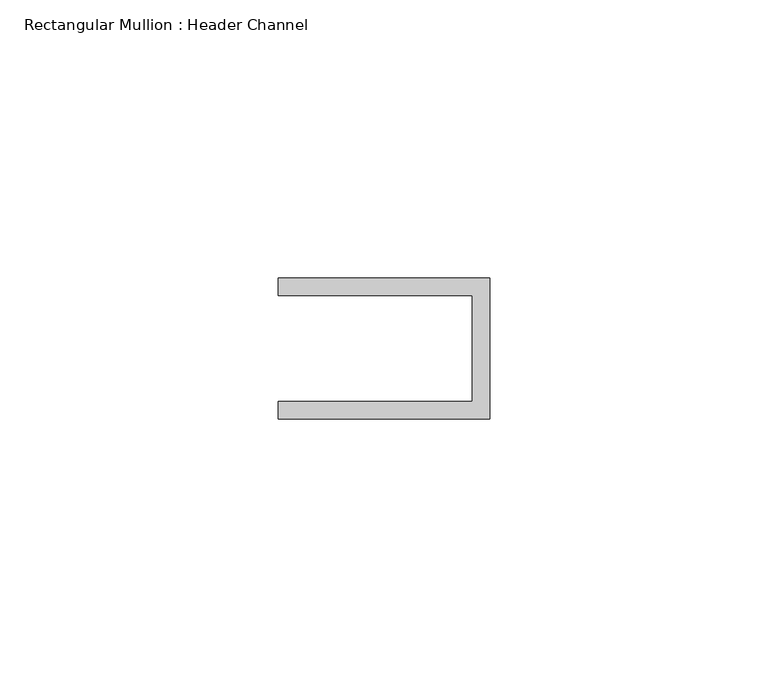
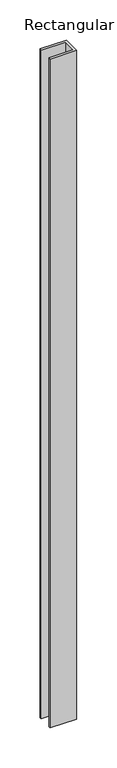
"""IFC4 building model written with IfcOpenShell, lengths in millimetres: member geometry, Rectangular Mullion : Header Channel."""

from ifc_helpers import new_model, si_unit, frame, origin, place, context, project, spatial, polyline, outline, extrude, source, transform, mapped, element, save


def rectangular_mullion_header_channel_3723cf62(model_context):
    return source(origin(), model_context, "Body", "SweptSolid", [
        extrude(outline(polyline([(0.0, -12.7), (-38.1, -12.7), (-38.1, -9.525), (-3.175, -9.525), (-3.175, 9.525), (-38.1, 9.525), (-38.1, 12.7), (0.0, 12.7), (0.0, -12.7)])), frame((0.0, 0.0, -1016.0), z_axis=(0.0, 0.0, 1.0), x_axis=(1.0, 0.0, 0.0)), (0.0, 0.0, 1.0), 1016.0),
    ])


if __name__ == "__main__":
    model = new_model("IFC4")
    model_context = context("Model", 3, world=origin())
    ifc_project = project(units=[si_unit("LENGTHUNIT", "METRE", prefix="MILLI")], contexts=[model_context])
    site = spatial("IfcSite", under=ifc_project)
    building = spatial("IfcBuilding", under=site)
    placement = place(None, origin())
    rectangular_mullion_header_channel_shape = rectangular_mullion_header_channel_3723cf62(model_context)
    element("IfcMember", 1, ObjectType="Rectangular Mullion : Header Channel", at=placement, inside=building, context=model_context, shape_type="MappedRepresentation", body=[
        mapped(rectangular_mullion_header_channel_shape, transform((0.0, 0.0, 0.0), x_axis=(1.0, 0.0, 0.0), y_axis=(0.0, 1.0, 0.0), z_axis=(0.0, 0.0, 1.0))),
    ])
    save(model, "model.ifc")

# Revit data of these elements
# Type "Rectangular Mullion : Header Channel"
#   built-in parameter 1007322 = 0.0833333 (stored number, unit not read)
#   built-in parameter 1007321 = -0.03125 (stored number, unit not read)
#   built-in parameter 1007320 = 0.0416667 (stored number, unit not read)
# Element 1 (IfcMember, "Rectangular Mullion : Header Channel")
#   Materials on its faces: "ALUM"
# Materials
#   "ALUM": class "Generic", colour RGB 157 157 157, transparency 0, Cost = 0
